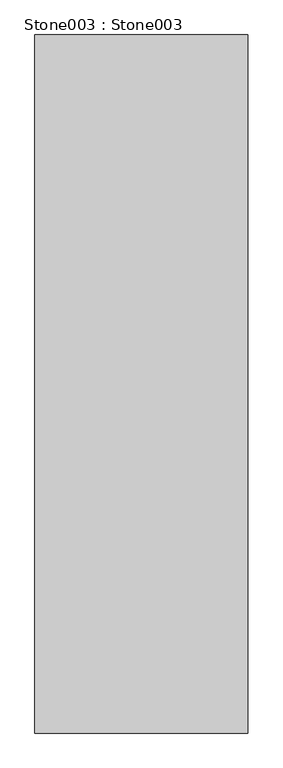
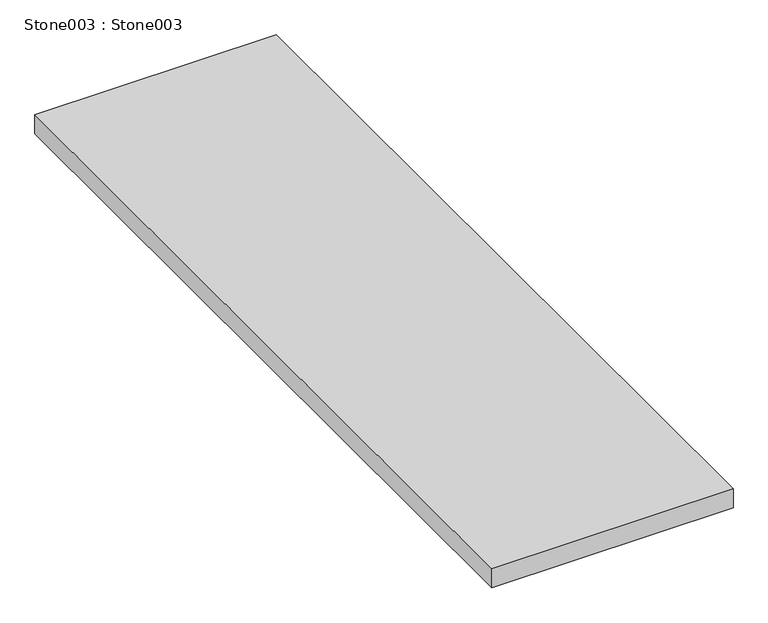
"""IFC4 building model written with IfcOpenShell, lengths in millimetres: proxy geometry, Stone003 : Stone003."""

from ifc_helpers import new_model, si_unit, frame, origin, place, context, project, spatial, polyline, outline, extrude, source, transform, mapped, element, save


def stone003_stone003_4f59213f(model_context):
    return source(origin(), model_context, "Body", "SweptSolid", [
        extrude(outline(polyline([(-2996.0543087, -1052.8906574), (-3605.6543087, -1052.8906574), (-3605.6543087, 947.1093426), (-2996.0543087, 947.1093426), (-2996.0543087, -1052.8906574)])), frame((0.0, 0.0, 36518.596), z_axis=(0.0, 0.0, 1.0), x_axis=(1.0, 0.0, 0.0)), (0.0, 0.0, 1.0), 50.8),
    ])


if __name__ == "__main__":
    model = new_model("IFC4")
    model_context = context("Model", 3, world=origin())
    ifc_project = project(units=[si_unit("LENGTHUNIT", "METRE", prefix="MILLI")], contexts=[model_context])
    site = spatial("IfcSite", under=ifc_project)
    building = spatial("IfcBuilding", under=site)
    placement = place(None, origin())
    stone003_stone003_shape = stone003_stone003_4f59213f(model_context)
    element("IfcBuildingElementProxy", 1, Name="Stone003 : Stone003", ObjectType="Stone003 : Stone003", at=placement, inside=building, context=model_context, shape_type="MappedRepresentation", body=[
        mapped(stone003_stone003_shape, transform((0.0, 0.0, 0.0), x_axis=(1.0, 0.0, 0.0), y_axis=(0.0, 1.0, 0.0), z_axis=(0.0, 0.0, 1.0))),
    ])
    save(model, "model.ifc")

# Revit data of these elements
# Type "Stone003 : Stone003"
#   NameOverride = "Stone003"
# Element 1 (IfcBuildingElementProxy, "Stone003 : Stone003")
#   Materials on its faces: "2\" STONE DECK TBD"
# Materials
#   "2\" STONE DECK TBD": class "Unassigned", colour RGB 199 185 173, transparency 0
